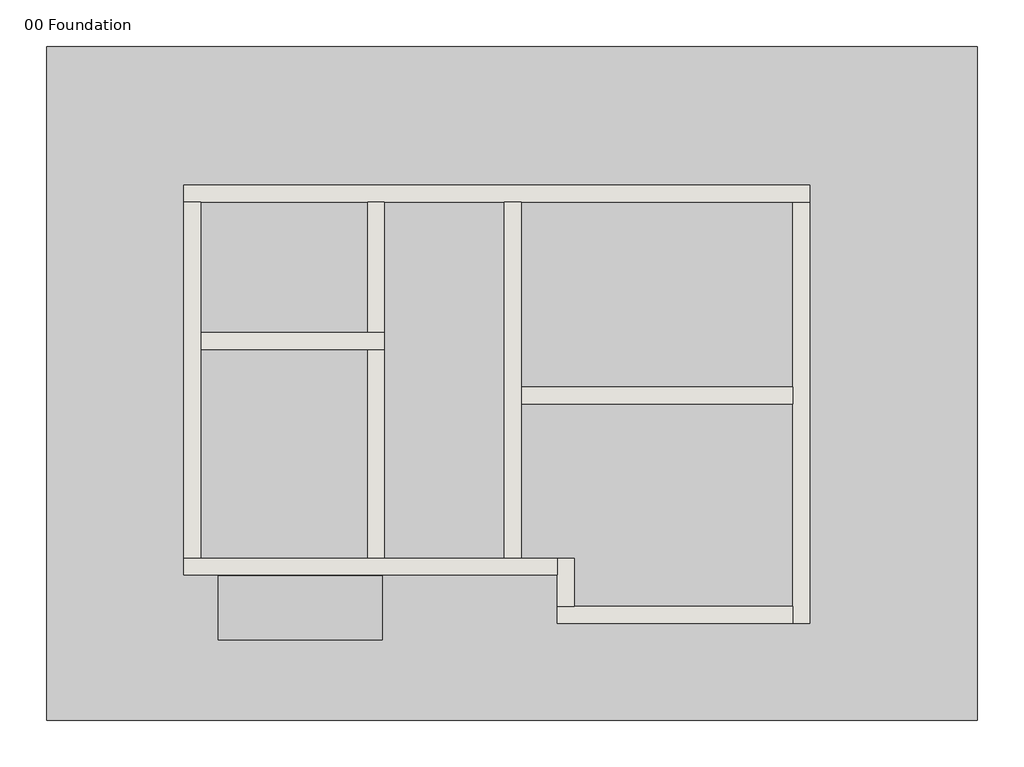
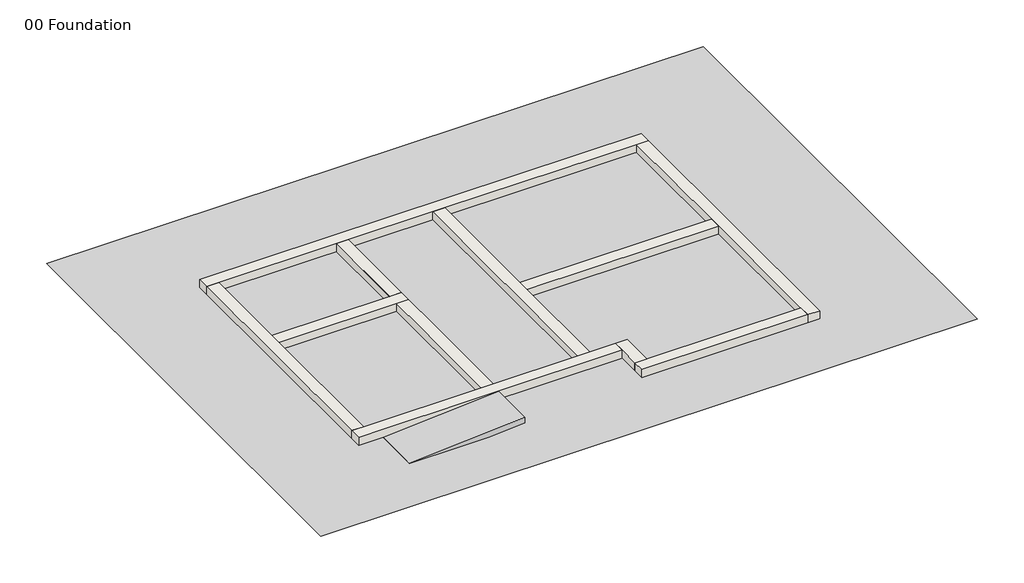
# One storey: 21 walls, 10 footings, 1 proxy, 1 ramp.
"""IFC4 building model written with IfcOpenShell, lengths in millimetres."""

import ifcopenshell
import ifcopenshell.guid

model = None  # the IFC model being written
_history = None  # IfcOwnerHistory: only IFC2X3 demands one
_inside = {}  # id of a spatial element -> (the spatial element, [elements in it])
_under = {}  # id of a project, library or spatial element -> (it, [spatial elements below it])
_declared = {}  # id of a project -> (the project, [libraries it declares])
_typed = {}  # id of a type object -> (the type object, [elements of that type])
_made_of = {}  # id of a material, layer set ... -> (it, [elements and type objects made of it])


def new_model(schema):
    """Start an empty IFC model of exactly this schema.

    Asked for "IFC4X3", IfcOpenShell would pick the latest addendum, in which some entities
    have other attributes; the version numbers below select the first issue.
    IFC2X3 requires an IfcOwnerHistory on every rooted entity: one is made here for all.
    """
    global model, _history
    if schema == "IFC4X3":
        model = ifcopenshell.file(schema_version=(4, 3, 0, 0))
    else:
        model = ifcopenshell.file(schema=schema)
    _inside.clear()
    _under.clear()
    _declared.clear()
    _typed.clear()
    _made_of.clear()
    _history = None
    if model.schema == "IFC2X3":
        org = make("IfcOrganization", Name="unknown")
        user = make(
            "IfcPersonAndOrganization",
            ThePerson=make("IfcPerson", FamilyName="unknown"),
            TheOrganization=org,
        )
        app = make(
            "IfcApplication",
            ApplicationDeveloper=org,
            Version="unknown",
            ApplicationFullName="unknown",
            ApplicationIdentifier="unknown",
        )
        _history = make(
            "IfcOwnerHistory",
            OwningUser=user,
            OwningApplication=app,
            ChangeAction="ADDED",
            CreationDate=0,
        )
    return model


def make(cls, **values):
    """One entity of the class cls with the attributes given. An attribute that is None is left unset."""
    return model.create_entity(
        cls, **{name: value for name, value in values.items() if value is not None}
    )


def rooted(cls, **values):
    """An entity with a GlobalId (a new one), such as an element, a storey or a relation."""
    return make(cls, GlobalId=ifcopenshell.guid.new(), OwnerHistory=_history, **values)


def si_unit(unit_type, name, prefix=None):
    """IfcSIUnit, for example si_unit("LENGTHUNIT", "METRE", prefix="MILLI")."""
    return make("IfcSIUnit", UnitType=unit_type, Prefix=prefix, Name=name)


def assignment(units):
    """IfcUnitAssignment: the units of a project."""
    return None if units is None else make("IfcUnitAssignment", Units=units)


def point(xyz):
    """IfcCartesianPoint."""
    return None if xyz is None else make("IfcCartesianPoint", Coordinates=xyz)


def direction(xyz):
    """IfcDirection."""
    return None if xyz is None else make("IfcDirection", DirectionRatios=xyz)


def frame(location, z_axis=None, x_axis=None):
    """IfcAxis2Placement3D, a coordinate frame: its origin and axes. An axis left out is left unset."""
    return make(
        "IfcAxis2Placement3D",
        Location=point(location),
        Axis=direction(z_axis),
        RefDirection=direction(x_axis),
    )


def origin():
    """The frame at (0, 0, 0) with its axes left unset."""
    return frame((0.0, 0.0, 0.0))


def place(relative_to, where):
    """IfcLocalPlacement: puts the frame where relative to a parent placement (None: the world)."""
    return make(
        "IfcLocalPlacement", PlacementRelTo=relative_to, RelativePlacement=where
    )


def context(
    kind, dimensions, precision=None, world=None, true_north=None, identifier=None
):
    """IfcGeometricRepresentationContext, for example the 3D "Model" context."""
    return make(
        "IfcGeometricRepresentationContext",
        ContextIdentifier=identifier,
        ContextType=kind,
        CoordinateSpaceDimension=dimensions,
        Precision=precision,
        WorldCoordinateSystem=world,
        TrueNorth=true_north,
    )


def project(units=None, contexts=None):
    """IfcProject with its units and contexts."""
    return rooted(
        "IfcProject",
        Name="project",
        RepresentationContexts=contexts,
        UnitsInContext=assignment(units),
    )


def spatial(cls, under=None, at=None, **own):
    """A site, building, storey or space (cls), placed at a placement, below another one or the project."""
    s = rooted(cls, ObjectPlacement=at, **own)
    if under is not None:
        _under.setdefault(under.id(), (under, []))[1].append(s)
    return s


def polyline(points):
    """IfcPolyline through the points."""
    return make("IfcPolyline", Points=[point(p) for p in points])


def point_list(points):
    """IfcCartesianPointList2D or 3D."""
    cls = (
        "IfcCartesianPointList2D" if len(points[0]) == 2 else "IfcCartesianPointList3D"
    )
    return make(cls, CoordList=points)


def outline(outer, holes=None, kind="AREA"):
    """IfcArbitraryClosedProfileDef: a profile drawn as a closed curve; with holes, ...WithVoids."""
    if holes is None:
        return make("IfcArbitraryClosedProfileDef", ProfileType=kind, OuterCurve=outer)
    return make(
        "IfcArbitraryProfileDefWithVoids",
        ProfileType=kind,
        OuterCurve=outer,
        InnerCurves=holes,
    )


def extrude(swept, where, along, depth):
    """IfcExtrudedAreaSolid: the profile swept, set in the frame where, extruded along a direction by depth."""
    return make(
        "IfcExtrudedAreaSolid",
        SweptArea=swept,
        Position=where,
        ExtrudedDirection=direction(along),
        Depth=depth,
    )


def faces_of(points, faces, orient=None, outer=None):
    """IfcFace entities. A face is a list of loops; a loop is a list of indices into points, from 0.

    orient and outer hold one flag for each loop. By default every Orientation is true, the
    first loop of a face is its IfcFaceOuterBound and the others are IfcFaceBound.
    """
    made = []
    for i, loops in enumerate(faces):
        bounds = []
        for j, loop in enumerate(loops):
            is_outer = j == 0 if outer is None else outer[i][j]
            bounds.append(
                make(
                    "IfcFaceOuterBound" if is_outer else "IfcFaceBound",
                    Bound=make("IfcPolyLoop", Polygon=[points[k] for k in loop]),
                    Orientation=True if orient is None else orient[i][j],
                )
            )
        made.append(make("IfcFace", Bounds=bounds))
    return made


def faceted_brep(points, faces, orient=None, outer=None, voids=None):
    """IfcFacetedBrep: a solid bounded by flat faces; with voids (closed shells), ...WithVoids."""
    shared = [point(p) for p in points]
    hull = make("IfcClosedShell", CfsFaces=faces_of(shared, faces, orient, outer))
    if voids is None:
        return make("IfcFacetedBrep", Outer=hull)
    return make(
        "IfcFacetedBrepWithVoids",
        Outer=hull,
        Voids=[
            make(cls, CfsFaces=faces_of(shared, fs, o, b)) for cls, fs, o, b in voids
        ],
    )


def triangles(points, corners, closed=None, point_numbers=None):
    """IfcTriangulatedFaceSet: each triangle names its three corners, points numbered from 1."""
    return make(
        "IfcTriangulatedFaceSet",
        Coordinates=point_list(points),
        Closed=closed,
        CoordIndex=corners,
        PnIndex=point_numbers,
    )


def shape(context_of_items, identifier, shape_type, items):
    """IfcShapeRepresentation: the items that make up one representation, for example the "Body"."""
    return make(
        "IfcShapeRepresentation",
        ContextOfItems=context_of_items,
        RepresentationIdentifier=identifier,
        RepresentationType=shape_type,
        Items=items,
    )


def source(mapping_origin, context_of_items, identifier, shape_type, items):
    """IfcRepresentationMap: a shape defined once, which mapped items show again and again."""
    return make(
        "IfcRepresentationMap",
        MappingOrigin=mapping_origin,
        MappedRepresentation=shape(context_of_items, identifier, shape_type, items),
    )


def transform(
    local_origin,
    x_axis=None,
    y_axis=None,
    z_axis=None,
    scale=None,
    scale2=None,
    scale3=None,
    uniform=True,
):
    """IfcCartesianTransformationOperator3D, or its non-uniform kind. x_axis, y_axis, z_axis: its Axis1, 2, 3."""
    if uniform:
        return make(
            "IfcCartesianTransformationOperator3D",
            Axis1=direction(x_axis),
            Axis2=direction(y_axis),
            LocalOrigin=point(local_origin),
            Scale=scale,
            Axis3=direction(z_axis),
        )
    return make(
        "IfcCartesianTransformationOperator3DnonUniform",
        Axis1=direction(x_axis),
        Axis2=direction(y_axis),
        LocalOrigin=point(local_origin),
        Scale=scale,
        Axis3=direction(z_axis),
        Scale2=scale2,
        Scale3=scale3,
    )


def mapped(mapping_source, mapping_target):
    """IfcMappedItem: shows the shape of a source again, moved by a transform."""
    return make(
        "IfcMappedItem", MappingSource=mapping_source, MappingTarget=mapping_target
    )


def made_of(thing, what):
    """Note that an element or type object is made of a material, layer set ...; save() writes the relation."""
    if what is not None:
        _made_of.setdefault(what.id(), (what, []))[1].append(thing)
    return thing


def element(
    cls,
    number,
    at=None,
    inside=None,
    cuts=None,
    type_object=None,
    material=None,
    context=None,
    identifier="Body",
    shape_type=None,
    held_by="IfcProductDefinitionShape",
    body=None,
    shapes=None,
    **own,
):
    """One element of the class cls, such as IfcWall. Its Tag is "e" and its number.

    at: its placement. inside: the storey or other place that contains it. cuts: it is an
    opening in that element (IfcRelVoidsElement). A single representation is given by context,
    identifier, shape_type and body (its items); several are given by shapes. held_by: the class
    of the entity that holds the representations. save() writes the other relations.
    """
    e = rooted(cls, Tag="e%d" % number, ObjectPlacement=at, **own)
    if body is not None:
        shapes = [shape(context, identifier, shape_type, body)]
    if shapes is not None:
        e.Representation = make(held_by, Representations=shapes)
    if inside is not None:
        _inside.setdefault(inside.id(), (inside, []))[1].append(e)
    if cuts is not None:
        rooted(
            "IfcRelVoidsElement", RelatingBuildingElement=cuts, RelatedOpeningElement=e
        )
    if type_object is not None:
        _typed.setdefault(type_object.id(), (type_object, []))[1].append(e)
    return made_of(e, material)


def aggregate(whole, parts):
    """IfcRelAggregates: a whole, such as a stair, and the parts it consists of."""
    return rooted("IfcRelAggregates", RelatingObject=whole, RelatedObjects=parts)


def save(model, path):
    """Write the relations noted so far, then the file.

    IfcRelAggregates (storeys below a building ...), IfcRelContainedInSpatialStructure (elements
    in a storey), IfcRelDefinesByType, IfcRelAssociatesMaterial and IfcRelDeclares: one each for
    every whole, place, type object, material and project.
    """
    for whole, parts in _under.values():
        aggregate(whole, parts)
    for where, things in _inside.values():
        rooted(
            "IfcRelContainedInSpatialStructure",
            RelatedElements=things,
            RelatingStructure=where,
        )
    for kind, things in _typed.values():
        rooted("IfcRelDefinesByType", RelatedObjects=things, RelatingType=kind)
    for what, things in _made_of.values():
        rooted("IfcRelAssociatesMaterial", RelatedObjects=things, RelatingMaterial=what)
    for by, libraries in _declared.values():
        rooted("IfcRelDeclares", RelatingContext=by, RelatedDefinitions=libraries)
    model.write(path)


def ramp_1_ce501800(model_context):
    return source(origin(), model_context, "Body", "SweptSolid", [
        extrude(outline(polyline([(0.0, -7500.2064028), (-225.0, -10560.2064028), (-375.4049465, -10560.2064028), (-150.4049465, -7500.2064028), (0.0, -7500.2064028)])), frame((0.0, -1636.162817, 0.0), z_axis=(0.0, 1.0, 0.0), x_axis=(0.0, 0.0, 1.0)), (0.0, 0.0, 1.0), 1200.0),
    ])


model = new_model("IFC4")

# Units and contexts
model_context = context("Model", 3, world=origin())
ifc_project = project(units=[si_unit("LENGTHUNIT", "METRE", prefix="MILLI")], contexts=[model_context])

# Site, building, storey
site = spatial("IfcSite", under=ifc_project)
building = spatial("IfcBuilding", under=site)
storey = spatial("IfcBuildingStorey", under=building, Name="00 Foundation", Elevation=-900.0)

# Proxy
placement = place(None, origin())
element("IfcBuildingElementProxy", 1, Name="Building Element Proxy", at=placement, inside=storey, context=model_context, shape_type="Tessellation", body=[
    triangles([(-13772.2558685, 9461.3562103, -225.0000017), (3627.7439735, 9461.3562103, -225.0000017), (3627.7439735, -3138.6435951, -225.0000017), (-13772.2558685, -3138.6435951, -225.0000017)], [[1, 4, 2], [3, 2, 4]], closed=False),
])

# Footings
element("IfcFooting", 2, ObjectType="Wall Foundation Domestic 910", at=placement, inside=storey, context=model_context, shape_type="Brep", body=[
    faceted_brep([(-10595.3997381, -720.6350684, -900.0), (-10595.3997381, 189.3649316, -900.0), (-10595.3997381, 3496.6149316, -900.0), (-10595.3997381, 4406.6149316, -900.0), (-10595.3997381, 6255.1149316, -900.0), (-10595.3997381, 7165.1149316, -900.0), (-11505.3997381, 7165.1149316, -900.0), (-11505.3997381, -720.6350684, -900.0), (-11505.3997381, -720.6350684, -1250.0), (-11505.3997381, 7165.1149316, -1250.0), (-10595.3997381, -720.6350684, -1250.0), (-10595.3997381, 7165.1149316, -1250.0), (-10595.3997381, 6255.1149316, -1250.0), (-10595.3997381, 4406.6149316, -1250.0), (-10595.3997381, 3496.6149316, -1250.0), (-10595.3997381, 189.3649316, -1250.0)], [[[0, 1, 2, 3, 4, 5, 6, 7]], [[8, 7, 6, 9]], [[10, 8, 9, 11, 12, 13, 14, 15]], [[0, 10, 15, 14, 13, 12, 11, 5, 4, 3, 2, 1]], [[6, 5, 11, 9]], [[0, 7, 8, 10]]]),
])
element("IfcFooting", 3, ObjectType="Wall Foundation Domestic 910", at=placement, inside=storey, context=model_context, shape_type="Brep", body=[
    faceted_brep([(792.3502619, 6255.1149316, -900.0), (792.3502619, 7165.1149316, -900.0), (-10595.3997381, 7165.1149316, -900.0), (-10595.3997381, 6255.1149316, -900.0), (-8069.2747381, 6255.1149316, -900.0), (-7159.2747381, 6255.1149316, -900.0), (-5512.2747381, 6255.1149316, -900.0), (-4602.2747381, 6255.1149316, -900.0), (-117.6497381, 6255.1149316, -900.0), (792.3502619, 7165.1149316, -1250.0), (-10595.3997381, 7165.1149316, -1250.0), (792.3502619, 6255.1149316, -1250.0), (-117.6497381, 6255.1149316, -1250.0), (-4602.2747381, 6255.1149316, -1250.0), (-5512.2747381, 6255.1149316, -1250.0), (-7159.2747381, 6255.1149316, -1250.0), (-8069.2747381, 6255.1149316, -1250.0), (-10595.3997381, 6255.1149316, -1250.0)], [[[0, 1, 2, 3, 4, 5, 6, 7, 8]], [[1, 9, 10, 2]], [[9, 11, 12, 13, 14, 15, 16, 17, 10]], [[11, 0, 8, 7, 6, 5, 4, 3, 17, 16, 15, 14, 13, 12]], [[3, 2, 10, 17]], [[1, 0, 11, 9]]]),
])
element("IfcFooting", 4, ObjectType="Wall Foundation Domestic 910", at=placement, inside=storey, context=model_context, shape_type="Brep", body=[
    faceted_brep([(-10595.3997381, 3496.6149316, -900.0), (-8069.2747381, 3496.6149316, -900.0), (-7159.2747381, 3496.6149316, -900.0), (-7159.2747381, 4406.6149316, -900.0), (-8069.2747381, 4406.6149316, -900.0), (-10595.3997381, 4406.6149316, -900.0), (-10595.3997381, 4406.6149316, -1250.0), (-7159.2747381, 4406.6149316, -1250.0), (-8069.2747381, 4406.6149316, -1250.0), (-10595.3997381, 3496.6149316, -1250.0), (-7159.2747381, 3496.6149316, -1250.0), (-8069.2747381, 3496.6149316, -1250.0)], [[[0, 1, 2, 3, 4, 5]], [[6, 5, 4, 3, 7, 8]], [[9, 6, 8, 7, 10, 11]], [[0, 9, 11, 10, 2, 1]], [[0, 5, 6, 9]], [[3, 2, 10, 7]]]),
])
element("IfcFooting", 5, ObjectType="Wall Foundation Domestic 910", at=placement, inside=storey, context=model_context, shape_type="SweptSolid", body=[
    extrude(outline(polyline([(-8069.2747381, 6255.1149316), (-7159.2747381, 6255.1149316), (-7159.2747381, 4406.6149316), (-8069.2747381, 4406.6149316), (-8069.2747381, 6255.1149316)])), frame((0.0, 0.0, -1250.0), z_axis=(0.0, 0.0, 1.0), x_axis=(1.0, 0.0, 0.0)), (0.0, 0.0, 1.0), 350.0),
    extrude(outline(polyline([(-7159.2747381, 189.3649316), (-8069.2747381, 189.3649316), (-8069.2747381, 3496.6149316), (-7159.2747381, 3496.6149316), (-7159.2747381, 189.3649316)])), frame((0.0, 0.0, -1250.0), z_axis=(0.0, 0.0, 1.0), x_axis=(1.0, 0.0, 0.0)), (0.0, 0.0, 1.0), 350.0),
])
element("IfcFooting", 6, ObjectType="Wall Foundation Domestic 910", at=placement, inside=storey, context=model_context, shape_type="Brep", body=[
    faceted_brep([(-5512.2747381, 6255.1149316, -900.0), (-5512.2747381, 189.3649316, -900.0), (-4602.2747381, 189.3649316, -900.0), (-4602.2747381, 2480.3649316, -900.0), (-4602.2747381, 3390.3649316, -900.0), (-4602.2747381, 6255.1149316, -900.0), (-4602.2747381, 6255.1149316, -1250.0), (-4602.2747381, 189.3649316, -1250.0), (-4602.2747381, 2480.3649316, -1250.0), (-4602.2747381, 3390.3649316, -1250.0), (-5512.2747381, 6255.1149316, -1250.0), (-5512.2747381, 189.3649316, -1250.0)], [[[0, 1, 2, 3, 4, 5]], [[6, 5, 4, 3, 2, 7, 8, 9]], [[10, 6, 9, 8, 7, 11]], [[0, 10, 11, 1]], [[0, 5, 6, 10]], [[2, 1, 11, 7]]]),
])
element("IfcFooting", 7, ObjectType="Wall Foundation Domestic 910", at=placement, inside=storey, context=model_context, shape_type="SweptSolid", body=[
    extrude(outline(polyline([(-117.6497381, 3390.3649316), (-117.6497381, 2480.3649316), (-4602.2747381, 2480.3649316), (-4602.2747381, 3390.3649316), (-117.6497381, 3390.3649316)])), frame((0.0, 0.0, -1250.0), z_axis=(0.0, 0.0, 1.0), x_axis=(1.0, 0.0, 0.0)), (0.0, 0.0, 1.0), 350.0),
])
element("IfcFooting", 8, ObjectType="Wall Foundation Domestic 910", at=placement, inside=storey, context=model_context, shape_type="Brep", body=[
    faceted_brep([(-117.6497381, -1620.6350684, -900.0), (792.3502619, -1620.6350684, -900.0), (792.3502619, 6255.1149316, -900.0), (-117.6497381, 6255.1149316, -900.0), (-117.6497381, 3390.3649316, -900.0), (-117.6497381, 2480.3649316, -900.0), (-117.6497381, -710.6350684, -900.0), (792.3502619, -1620.6350684, -1250.0), (792.3502619, 6255.1149316, -1250.0), (-117.6497381, -1620.6350684, -1250.0), (-117.6497381, -710.6350684, -1250.0), (-117.6497381, 2480.3649316, -1250.0), (-117.6497381, 3390.3649316, -1250.0), (-117.6497381, 6255.1149316, -1250.0)], [[[0, 1, 2, 3, 4, 5, 6]], [[1, 7, 8, 2]], [[7, 9, 10, 11, 12, 13, 8]], [[9, 0, 6, 5, 4, 3, 13, 12, 11, 10]], [[3, 2, 8, 13]], [[1, 0, 9, 7]]]),
])
element("IfcFooting", 9, ObjectType="Wall Foundation Domestic 910", at=placement, inside=storey, context=model_context, shape_type="Brep", body=[
    faceted_brep([(-3609.7747381, -720.6350684, -900.0), (-3609.7747381, -710.6350684, -900.0), (-3609.7747381, 189.3649316, -900.0), (-4602.2747381, 189.3649316, -900.0), (-5512.2747381, 189.3649316, -900.0), (-7159.2747381, 189.3649316, -900.0), (-8069.2747381, 189.3649316, -900.0), (-10595.3997381, 189.3649316, -900.0), (-10595.3997381, -720.6350684, -900.0), (-4519.7747381, -720.6350684, -900.0), (-3609.7747381, -720.6350684, -1250.0), (-10595.3997381, -720.6350684, -1250.0), (-4519.7747381, -720.6350684, -1250.0), (-3609.7747381, 189.3649316, -1250.0), (-3609.7747381, -710.6350684, -1250.0), (-10595.3997381, 189.3649316, -1250.0), (-8069.2747381, 189.3649316, -1250.0), (-7159.2747381, 189.3649316, -1250.0), (-5512.2747381, 189.3649316, -1250.0), (-4602.2747381, 189.3649316, -1250.0)], [[[0, 1, 2, 3, 4, 5, 6, 7, 8, 9]], [[10, 0, 9, 8, 11, 12]], [[13, 14, 10, 12, 11, 15, 16, 17, 18, 19]], [[2, 13, 19, 18, 17, 16, 15, 7, 6, 5, 4, 3]], [[8, 7, 15, 11]], [[2, 1, 0, 10, 14, 13]]]),
])
element("IfcFooting", 10, ObjectType="Wall Foundation Domestic 910", at=placement, inside=storey, context=model_context, shape_type="SweptSolid", body=[
    extrude(outline(polyline([(-3609.7747381, -1620.6350684), (-4519.7747381, -1620.6350684), (-4519.7747381, -720.6350684), (-3609.7747381, -720.6350684), (-3609.7747381, -1620.6350684)])), frame((0.0, 0.0, -1250.0), z_axis=(0.0, 0.0, 1.0), x_axis=(1.0, 0.0, 0.0)), (0.0, 0.0, 1.0), 350.0),
])
element("IfcFooting", 11, ObjectType="Wall Foundation Domestic 910", at=placement, inside=storey, context=model_context, shape_type="Brep", body=[
    faceted_brep([(-117.6497381, -1620.6350684, -900.0), (-117.6497381, -710.6350684, -900.0), (-3609.7747381, -710.6350684, -900.0), (-3609.7747381, -720.6350684, -900.0), (-3609.7747381, -1620.6350684, -900.0), (-117.6497381, -1620.6350684, -1250.0), (-3609.7747381, -1620.6350684, -1250.0), (-117.6497381, -710.6350684, -1250.0), (-3609.7747381, -720.6350684, -1250.0), (-3609.7747381, -710.6350684, -1250.0)], [[[0, 1, 2, 3, 4]], [[5, 0, 4, 6]], [[7, 5, 6, 8, 9]], [[1, 7, 9, 2]], [[1, 0, 5, 7]], [[2, 9, 8, 6, 4, 3]]]),
])

# Ramp
ramp_1_shape = ramp_1_ce501800(model_context)
element("IfcRamp", 12, ObjectType="Ramp 1", at=placement, inside=storey, context=model_context, shape_type="MappedRepresentation", body=[
    mapped(ramp_1_shape, transform((0.0, 0.0, 0.0), x_axis=(1.0, 0.0, 0.0), y_axis=(0.0, 1.0, 0.0), z_axis=(0.0, 0.0, 1.0))),
])

# Walls
element("IfcWall", 13, ObjectType="EF_20_05_Wall-Fnd_440DBlk (Trench Blockwork)", at=placement, inside=storey, context=model_context, shape_type="Brep", body=[
    faceted_brep([(-10830.3997381, -45.6350684, -900.0), (-10830.3997381, 3731.6149316, -900.0), (-10830.3997381, 4171.6149316, -900.0), (-10830.3997381, 6490.1149316, -900.0), (-10830.3997381, 6930.1149316, -900.0), (-10830.3997381, 6930.1149316, -450.0), (-10830.3997381, 6490.1149316, -450.0), (-10830.3997381, 4171.6149316, -450.0), (-10830.3997381, 3731.6149316, -450.0), (-10830.3997381, -45.6350684, -450.0), (-11270.3997381, -45.6350684, -900.0), (-11270.3997381, -45.6350684, -450.0), (-11270.3997381, 6930.1149316, -450.0), (-11270.3997381, 6930.1149316, -900.0)], [[[0, 1, 2, 3, 4, 5, 6, 7, 8, 9]], [[10, 11, 12, 13]], [[4, 3, 2, 1, 0, 10, 13]], [[9, 8, 7, 6, 5, 12, 11]], [[5, 4, 13, 12]], [[0, 9, 11, 10]]]),
])
element("IfcWall", 14, ObjectType="EF_20_05_Wall-Fnd_440DBlk (Trench Blockwork)", at=placement, inside=storey, context=model_context, shape_type="Brep", body=[
    faceted_brep([(-10830.3997381, 6490.1149316, -900.0), (-7834.2747381, 6490.1149316, -900.0), (-7394.2747381, 6490.1149316, -900.0), (-5277.2747381, 6490.1149316, -900.0), (-4837.2747381, 6490.1149316, -900.0), (117.3502619, 6490.1149316, -900.0), (557.3502619, 6490.1149316, -900.0), (557.3502619, 6490.1149316, -450.0), (117.3502619, 6490.1149316, -450.0), (-4837.2747381, 6490.1149316, -450.0), (-5277.2747381, 6490.1149316, -450.0), (-7394.2747381, 6490.1149316, -450.0), (-7834.2747381, 6490.1149316, -450.0), (-10830.3997381, 6490.1149316, -450.0), (-10830.3997381, 6930.1149316, -900.0), (-10830.3997381, 6930.1149316, -450.0), (557.3502619, 6930.1149316, -450.0), (557.3502619, 6930.1149316, -900.0)], [[[0, 1, 2, 3, 4, 5, 6, 7, 8, 9, 10, 11, 12, 13]], [[14, 15, 16, 17]], [[6, 5, 4, 3, 2, 1, 0, 14, 17]], [[13, 12, 11, 10, 9, 8, 7, 16, 15]], [[0, 13, 15, 14]], [[7, 6, 17, 16]]]),
])
element("IfcWall", 15, ObjectType="EF_20_05_Wall-Fnd_440DBlk (Trench Blockwork)", at=placement, inside=storey, context=model_context, shape_type="Brep", body=[
    faceted_brep([(117.3502619, 6490.1149316, -900.0), (117.3502619, 3155.3649316, -900.0), (117.3502619, 2715.3649316, -900.0), (117.3502619, -945.6350684, -900.0), (117.3502619, -1385.6350684, -900.0), (117.3502619, -1385.6350684, -450.0), (117.3502619, -945.6350684, -450.0), (117.3502619, 2715.3649316, -450.0), (117.3502619, 3155.3649316, -450.0), (117.3502619, 6490.1149316, -450.0), (557.3502619, 6490.1149316, -900.0), (557.3502619, 6490.1149316, -450.0), (557.3502619, -1385.6350684, -450.0), (557.3502619, -1385.6350684, -900.0)], [[[0, 1, 2, 3, 4, 5, 6, 7, 8, 9]], [[10, 11, 12, 13]], [[4, 3, 2, 1, 0, 10, 13]], [[9, 8, 7, 6, 5, 12, 11]], [[5, 4, 13, 12]], [[0, 9, 11, 10]]]),
])
element("IfcWall", 16, ObjectType="EF_20_05_Wall-Fnd_440DBlk (Trench Blockwork)", at=placement, inside=storey, context=model_context, shape_type="Brep", body=[
    faceted_brep([(-4284.7747381, -45.6350684, -900.0), (-4837.2747381, -45.6350684, -900.0), (-5277.2747381, -45.6350684, -900.0), (-7394.2747381, -45.6350684, -900.0), (-7834.2747381, -45.6350684, -900.0), (-10830.3997381, -45.6350684, -900.0), (-11270.3997381, -45.6350684, -900.0), (-11270.3997381, -45.6350684, -450.0), (-10830.3997381, -45.6350684, -450.0), (-7834.2747381, -45.6350684, -450.0), (-7394.2747381, -45.6350684, -450.0), (-5277.2747381, -45.6350684, -450.0), (-4837.2747381, -45.6350684, -450.0), (-4284.7747381, -45.6350684, -450.0), (-4284.7747381, -485.6350684, -900.0), (-4284.7747381, -485.6350684, -450.0), (-11270.3997381, -485.6350684, -450.0), (-11270.3997381, -485.6350684, -900.0)], [[[0, 1, 2, 3, 4, 5, 6, 7, 8, 9, 10, 11, 12, 13]], [[14, 15, 16, 17]], [[6, 5, 4, 3, 2, 1, 0, 14, 17]], [[13, 12, 11, 10, 9, 8, 7, 16, 15]], [[7, 6, 17, 16]], [[0, 13, 15, 14]]]),
])
element("IfcWall", 17, ObjectType="EF_20_05_Wall-Fnd_440DBlk (Trench Blockwork)", at=placement, inside=storey, context=model_context, shape_type="SweptSolid", body=[
    extrude(outline(polyline([(-3844.7747381, -945.6350684), (117.3502619, -945.6350684), (117.3502619, -1385.6350684), (-3844.7747381, -1385.6350684), (-3844.7747381, -945.6350684)])), frame((0.0, 0.0, -900.0), z_axis=(0.0, 0.0, 1.0), x_axis=(1.0, 0.0, 0.0)), (0.0, 0.0, 1.0), 450.0),
])
element("IfcWall", 18, ObjectType="EF_20_05_Wall-Fnd_440DBlk (Trench Blockwork)", at=placement, inside=storey, context=model_context, shape_type="Brep", body=[
    faceted_brep([(-3844.7747381, -1385.6350684, -900.0), (-3844.7747381, -945.6350684, -900.0), (-3844.7747381, -45.6350684, -900.0), (-3844.7747381, -45.6350684, -450.0), (-3844.7747381, -945.6350684, -450.0), (-3844.7747381, -1385.6350684, -450.0), (-4284.7747381, -1385.6350684, -900.0), (-4284.7747381, -1385.6350684, -450.0), (-4284.7747381, -485.6350684, -450.0), (-4284.7747381, -45.6350684, -450.0), (-4284.7747381, -45.6350684, -900.0), (-4284.7747381, -485.6350684, -900.0)], [[[0, 1, 2, 3, 4, 5]], [[6, 7, 8, 9, 10, 11]], [[2, 1, 0, 6, 11, 10]], [[5, 4, 3, 9, 8, 7]], [[3, 2, 10, 9]], [[0, 5, 7, 6]]]),
])
element("IfcWall", 19, ObjectType="EF_20_05_Wall-Fnd_440DBlk (Trench Blockwork)", at=placement, inside=storey, context=model_context, shape_type="SweptSolid", body=[
    extrude(outline(polyline([(-7834.2747381, 3731.6149316), (-10830.3997381, 3731.6149316), (-10830.3997381, 4171.6149316), (-7834.2747381, 4171.6149316), (-7834.2747381, 3731.6149316)])), frame((0.0, 0.0, -900.0), z_axis=(0.0, 0.0, 1.0), x_axis=(1.0, 0.0, 0.0)), (0.0, 0.0, 1.0), 450.0),
])
element("IfcWall", 20, ObjectType="EF_20_05_Wall-Fnd_440DBlk (Trench Blockwork)", at=placement, inside=storey, context=model_context, shape_type="Brep", body=[
    faceted_brep([(-7394.2747381, -45.6350684, -900.0), (-7394.2747381, 6490.1149316, -900.0), (-7394.2747381, 6490.1149316, -450.0), (-7394.2747381, -45.6350684, -450.0), (-7834.2747381, -45.6350684, -900.0), (-7834.2747381, -45.6350684, -450.0), (-7834.2747381, 3731.6149316, -450.0), (-7834.2747381, 4171.6149316, -450.0), (-7834.2747381, 6490.1149316, -450.0), (-7834.2747381, 6490.1149316, -900.0), (-7834.2747381, 4171.6149316, -900.0), (-7834.2747381, 3731.6149316, -900.0)], [[[0, 1, 2, 3]], [[4, 5, 6, 7, 8, 9, 10, 11]], [[1, 0, 4, 11, 10, 9]], [[3, 2, 8, 7, 6, 5]], [[2, 1, 9, 8]], [[0, 3, 5, 4]]]),
])
element("IfcWall", 21, ObjectType="EF_20_05_Wall-Fnd_440DBlk (Trench Blockwork)", at=placement, inside=storey, context=model_context, shape_type="Brep", body=[
    faceted_brep([(-5277.2747381, 6490.1149316, -900.0), (-5277.2747381, -45.6350684, -900.0), (-5277.2747381, -45.6350684, -450.0), (-5277.2747381, 6490.1149316, -450.0), (-4837.2747381, 6490.1149316, -900.0), (-4837.2747381, 6490.1149316, -450.0), (-4837.2747381, 3155.3649316, -450.0), (-4837.2747381, 2715.3649316, -450.0), (-4837.2747381, -45.6350684, -450.0), (-4837.2747381, -45.6350684, -900.0), (-4837.2747381, 2715.3649316, -900.0), (-4837.2747381, 3155.3649316, -900.0)], [[[0, 1, 2, 3]], [[4, 5, 6, 7, 8, 9, 10, 11]], [[1, 0, 4, 11, 10, 9]], [[3, 2, 8, 7, 6, 5]], [[0, 3, 5, 4]], [[2, 1, 9, 8]]]),
])
element("IfcWall", 22, ObjectType="EF_20_05_Wall-Fnd_440DBlk (Trench Blockwork)", at=placement, inside=storey, context=model_context, shape_type="SweptSolid", body=[
    extrude(outline(polyline([(117.3502619, 2715.3649316), (-4837.2747381, 2715.3649316), (-4837.2747381, 3155.3649316), (117.3502619, 3155.3649316), (117.3502619, 2715.3649316)])), frame((0.0, 0.0, -900.0), z_axis=(0.0, 0.0, 1.0), x_axis=(1.0, 0.0, 0.0)), (0.0, 0.0, 1.0), 450.0),
])
element("IfcWall", 23, ObjectType="EF_25_10_25_Wall-Ext-Cav_100Blk-115Conc-100Blk", at=placement, inside=storey, context=model_context, shape_type="Brep", body=[
    faceted_brep([(-11207.8997381, 6552.6149316, -450.0), (-10892.8997381, 6552.6149316, -450.0), (-7771.7747381, 6552.6149316, -450.0), (-7456.7747381, 6552.6149316, -450.0), (-5214.7747381, 6552.6149316, -450.0), (-4899.7747381, 6552.6149316, -450.0), (179.8502619, 6552.6149316, -450.0), (494.8502619, 6552.6149316, -450.0), (494.8502619, 6552.6149316, 0.0), (179.8502619, 6552.6149316, 0.0), (-4899.7747381, 6552.6149316, 0.0), (-5214.7747381, 6552.6149316, 0.0), (-7456.7747381, 6552.6149316, 0.0), (-7771.7747381, 6552.6149316, 0.0), (-10892.8997381, 6552.6149316, 0.0), (-11207.8997381, 6552.6149316, 0.0), (-11207.8997381, 6867.6149316, -450.0), (-11207.8997381, 6867.6149316, 0.0), (494.8502619, 6867.6149316, 0.0), (494.8502619, 6867.6149316, -450.0)], [[[0, 1, 2, 3, 4, 5, 6, 7, 8, 9, 10, 11, 12, 13, 14, 15]], [[16, 17, 18, 19]], [[7, 6, 5, 4, 3, 2, 1, 0, 16, 19]], [[15, 14, 13, 12, 11, 10, 9, 8, 18, 17]], [[8, 7, 19, 18]], [[0, 15, 17, 16]]]),
])
element("IfcWall", 24, ObjectType="EF_25_10_25_Wall-Ext-Cav_100Blk-115Conc-100Blk", at=placement, inside=storey, context=model_context, shape_type="Brep", body=[
    faceted_brep([(179.8502619, 6552.6149316, -450.0), (179.8502619, 3092.8649316, -450.0), (179.8502619, 2777.8649316, -450.0), (179.8502619, -1008.1350684, -450.0), (179.8502619, -1323.1350684, -450.0), (179.8502619, -1323.1350684, 0.0), (179.8502619, -1008.1350684, 0.0), (179.8502619, 2777.8649316, 0.0), (179.8502619, 3092.8649316, 0.0), (179.8502619, 6552.6149316, 0.0), (494.8502619, 6552.6149316, -450.0), (494.8502619, 6552.6149316, 0.0), (494.8502619, -1323.1350684, 0.0), (494.8502619, -1323.1350684, -450.0)], [[[0, 1, 2, 3, 4, 5, 6, 7, 8, 9]], [[10, 11, 12, 13]], [[4, 3, 2, 1, 0, 10, 13]], [[9, 8, 7, 6, 5, 12, 11]], [[0, 9, 11, 10]], [[5, 4, 13, 12]]]),
])
element("IfcWall", 25, ObjectType="EF_25_10_25_Wall-Ext-Cav_100Blk-115Conc-100Blk", at=placement, inside=storey, context=model_context, shape_type="Brep", body=[
    faceted_brep([(179.8502619, -1008.1350684, -450.0), (-3907.2747381, -1008.1350684, -450.0), (-4222.2747381, -1008.1350684, -450.0), (-4222.2747381, -1008.1350684, 0.0), (-3907.2747381, -1008.1350684, 0.0), (179.8502619, -1008.1350684, 0.0), (179.8502619, -1323.1350684, -450.0), (179.8502619, -1323.1350684, 0.0), (-4222.2747381, -1323.1350684, 0.0), (-4222.2747381, -1323.1350684, -450.0)], [[[0, 1, 2, 3, 4, 5]], [[6, 7, 8, 9]], [[2, 1, 0, 6, 9]], [[5, 4, 3, 8, 7]], [[0, 5, 7, 6]], [[3, 2, 9, 8]]]),
])
element("IfcWall", 26, ObjectType="EF_25_10_25_Wall-Ext-Cav_100Blk-115Conc-100Blk", at=placement, inside=storey, context=model_context, shape_type="Brep", body=[
    faceted_brep([(-3907.2747381, -1008.1350684, -450.0), (-3907.2747381, -108.1350684, -450.0), (-3907.2747381, -108.1350684, 0.0), (-3907.2747381, -1008.1350684, 0.0), (-4222.2747381, -1008.1350684, -450.0), (-4222.2747381, -1008.1350684, 0.0), (-4222.2747381, -423.1350684, 0.0), (-4222.2747381, -108.1350684, 0.0), (-4222.2747381, -108.1350684, -450.0), (-4222.2747381, -423.1350684, -450.0)], [[[0, 1, 2, 3]], [[4, 5, 6, 7, 8, 9]], [[1, 0, 4, 9, 8]], [[3, 2, 7, 6, 5]], [[0, 3, 5, 4]], [[2, 1, 8, 7]]]),
])
element("IfcWall", 27, ObjectType="EF_25_10_25_Wall-Ext-Cav_100Blk-115Conc-100Blk", at=placement, inside=storey, context=model_context, shape_type="Brep", body=[
    faceted_brep([(-4222.2747381, -108.1350684, -450.0), (-4899.7747381, -108.1350684, -450.0), (-5214.7747381, -108.1350684, -450.0), (-7456.7747381, -108.1350684, -450.0), (-7771.7747381, -108.1350684, -450.0), (-10892.8997381, -108.1350684, -450.0), (-11207.8997381, -108.1350684, -450.0), (-11207.8997381, -108.1350684, 0.0), (-10892.8997381, -108.1350684, 0.0), (-7771.7747381, -108.1350684, 0.0), (-7456.7747381, -108.1350684, 0.0), (-5214.7747381, -108.1350684, 0.0), (-4899.7747381, -108.1350684, 0.0), (-4222.2747381, -108.1350684, 0.0), (-4222.2747381, -423.1350684, -450.0), (-4222.2747381, -423.1350684, 0.0), (-11207.8997381, -423.1350684, 0.0), (-11207.8997381, -423.1350684, -450.0)], [[[0, 1, 2, 3, 4, 5, 6, 7, 8, 9, 10, 11, 12, 13]], [[14, 15, 16, 17]], [[6, 5, 4, 3, 2, 1, 0, 14, 17]], [[13, 12, 11, 10, 9, 8, 7, 16, 15]], [[0, 13, 15, 14]], [[7, 6, 17, 16]]]),
])
element("IfcWall", 28, ObjectType="EF_25_10_25_Wall-Ext-Cav_100Blk-115Conc-100Blk", at=placement, inside=storey, context=model_context, shape_type="Brep", body=[
    faceted_brep([(-10892.8997381, -108.1350684, -450.0), (-10892.8997381, 3794.1149316, -450.0), (-10892.8997381, 4109.1149316, -450.0), (-10892.8997381, 6552.6149316, -450.0), (-10892.8997381, 6552.6149316, 0.0), (-10892.8997381, 4109.1149316, 0.0), (-10892.8997381, 3794.1149316, 0.0), (-10892.8997381, -108.1350684, 0.0), (-11207.8997381, -108.1350684, -450.0), (-11207.8997381, -108.1350684, 0.0), (-11207.8997381, 6552.6149316, 0.0), (-11207.8997381, 6552.6149316, -450.0)], [[[0, 1, 2, 3, 4, 5, 6, 7]], [[8, 9, 10, 11]], [[3, 2, 1, 0, 8, 11]], [[7, 6, 5, 4, 10, 9]], [[0, 7, 9, 8]], [[4, 3, 11, 10]]]),
])
element("IfcWall", 29, ObjectType="EF_25_10_25_Wall-Ext-Cav_100Blk-115Conc-100Blk", at=placement, inside=storey, context=model_context, shape_type="Brep", body=[
    faceted_brep([(-10892.8997381, 3794.1149316, -450.0), (-7456.7747381, 3794.1149316, -450.0), (-7456.7747381, 3794.1149316, 0.0), (-10892.8997381, 3794.1149316, 0.0), (-10892.8997381, 4109.1149316, -450.0), (-10892.8997381, 4109.1149316, 0.0), (-7771.7747381, 4109.1149316, 0.0), (-7456.7747381, 4109.1149316, 0.0), (-7456.7747381, 4109.1149316, -450.0), (-7771.7747381, 4109.1149316, -450.0)], [[[0, 1, 2, 3]], [[4, 5, 6, 7, 8, 9]], [[1, 0, 4, 9, 8]], [[3, 2, 7, 6, 5]], [[0, 3, 5, 4]], [[2, 1, 8, 7]]]),
])
element("IfcWall", 30, ObjectType="EF_25_10_25_Wall-Ext-Cav_100Blk-115Conc-100Blk", at=placement, inside=storey, context=model_context, shape_type="SweptSolid", body=[
    extrude(outline(polyline([(-7456.7747381, 6552.6149316), (-7456.7747381, 4109.1149316), (-7771.7747381, 4109.1149316), (-7771.7747381, 6552.6149316), (-7456.7747381, 6552.6149316)])), frame((0.0, 0.0, -450.0), z_axis=(0.0, 0.0, 1.0), x_axis=(1.0, 0.0, 0.0)), (0.0, 0.0, 1.0), 450.0),
])
element("IfcWall", 31, ObjectType="EF_25_10_25_Wall-Ext-Cav_100Blk-115Conc-100Blk", at=placement, inside=storey, context=model_context, shape_type="SweptSolid", body=[
    extrude(outline(polyline([(-7771.7747381, -108.1350684), (-7771.7747381, 6552.6149316), (-7456.7747381, 6552.6149316), (-7456.7747381, -108.1350684), (-7771.7747381, -108.1350684)])), frame((0.0, 0.0, -450.0), z_axis=(0.0, 0.0, 1.0), x_axis=(1.0, 0.0, 0.0)), (0.0, 0.0, 1.0), 450.0),
])
element("IfcWall", 32, ObjectType="EF_25_10_25_Wall-Ext-Cav_100Blk-115Conc-100Blk", at=placement, inside=storey, context=model_context, shape_type="Brep", body=[
    faceted_brep([(-5214.7747381, 6552.6149316, -450.0), (-5214.7747381, -108.1350684, -450.0), (-5214.7747381, -108.1350684, 0.0), (-5214.7747381, 6552.6149316, 0.0), (-4899.7747381, 6552.6149316, -450.0), (-4899.7747381, 6552.6149316, 0.0), (-4899.7747381, 3092.8649316, 0.0), (-4899.7747381, 2777.8649316, 0.0), (-4899.7747381, -108.1350684, 0.0), (-4899.7747381, -108.1350684, -450.0), (-4899.7747381, 2777.8649316, -450.0), (-4899.7747381, 3092.8649316, -450.0)], [[[0, 1, 2, 3]], [[4, 5, 6, 7, 8, 9, 10, 11]], [[1, 0, 4, 11, 10, 9]], [[3, 2, 8, 7, 6, 5]], [[0, 3, 5, 4]], [[2, 1, 9, 8]]]),
])
element("IfcWall", 33, ObjectType="EF_25_10_25_Wall-Ext-Cav_100Blk-115Conc-100Blk", at=placement, inside=storey, context=model_context, shape_type="SweptSolid", body=[
    extrude(outline(polyline([(179.8502619, 2777.8649316), (-4899.7747381, 2777.8649316), (-4899.7747381, 3092.8649316), (179.8502619, 3092.8649316), (179.8502619, 2777.8649316)])), frame((0.0, 0.0, -450.0), z_axis=(0.0, 0.0, 1.0), x_axis=(1.0, 0.0, 0.0)), (0.0, 0.0, 1.0), 450.0),
])

save(model, "model.ifc")

# Revit data of these elements
# Project information
#   Document_Suitability_Code = "P2"
#   Document_Suitability_Description = "Coordination"
#   Project Issue Date = "22-Feb-23"
#   Project Status = "Project Status"
#   Client Name = "Revit Project"
#   Project Address = "Enter address here"
#   Project Name = "Two Storey House"
#   Project Number = "CADD06021-01"
# Type "Ramp 1"
#   built-in parameter 1008304 = 0.492126 (stored number, unit not read)
#   built-in parameter 1008303 = 39.3701 (stored number, unit not read)
#   built-in parameter 1008301 = 12 (stored number, unit not read)
#   Function = 1
#   built-in parameter 1008308 = Concrete, Cast In Situ
# Type "EF_20_05_Wall-Fnd_440DBlk (Trench Blockwork)"
#   Keynote = "F10"
#   Layers, outside or top first: 440 mm "Concrete Masonry Units 440" (function 1)
# Type "EF_25_10_25_Wall-Ext-Cav_100Blk-115Conc-100Blk"
#   Keynote = "F10"
#   Layers, outside or top first: 100 mm "Concrete Masonry Units" (function 4); 115 mm "Concrete, Cast In Situ" (function 3); 100 mm "Concrete Masonry Units" (function 1)
# Element 1 (IfcBuildingElementProxy)
#   Material = Earth
#   Phase Created = New Construction
# Elements 2, 3, 4, 5, 6, 7, 8, 9, 10, 11 (IfcFooting, "Wall Foundation Domestic 910")
#   Comments = ""
#   Phase Created = New Construction
#   Materials on its faces: "Concrete, Cast In Situ"
# Element 12 (IfcRamp, "Ramp 1")
#   built-in parameter 1007275 = "DN"
#   built-in parameter 1007272 = "UP"
#   built-in parameter 1007218 = -0.738189 (stored number, unit not read)
#   Width = 1200 mm
#   built-in parameter 1007276 = 1
#   built-in parameter 1007274 = 1
#   built-in parameter 1007273 = 1
#   built-in parameter 1007271 = 1
#   Phase Created = New Construction
#   Materials on its faces: "Concrete, Cast In Situ"
# Elements 13, 14, 15, 16, 17, 18, 19, 20, 21, 22 (IfcWall, "EF_20_05_Wall-Fnd_440DBlk (Trench Blockwork)")
#   Top Offset = -450 mm
#   Base Offset = 0 mm
#   wall height = 450 mm
#   Phase Created = New Construction
#   Base Constraint = 00 Foundation
#   Top Constraint = 00 Ground Floor
#   Materials on its faces: "Concrete Masonry Units 440"
# Elements 23, 24, 25, 26, 27, 29 (IfcWall, "EF_25_10_25_Wall-Ext-Cav_100Blk-115Conc-100Blk")
#   built-in parameter 1001111 = 450 mm
#   Top Offset = 0 mm
#   Base Offset = 450 mm
#   wall height = 450 mm
#   Phase Created = New Construction
#   Base Constraint = 00 Foundation
#   Top Constraint = 00 Ground Floor
#   Materials on its faces: "Concrete Masonry Units", "Default Wall"
# Elements 28, 30, 31, 32, 33 (IfcWall, "EF_25_10_25_Wall-Ext-Cav_100Blk-115Conc-100Blk")
#   built-in parameter 1001111 = 450 mm
#   Top Offset = 0 mm
#   Base Offset = 450 mm
#   wall height = 450 mm
#   Phase Created = New Construction
#   Base Constraint = 00 Foundation
#   Top Constraint = 00 Ground Floor
#   Materials on its faces: "Default Wall", "Concrete Masonry Units"
# Materials
#   "Concrete, Cast In Situ": class "Concrete", colour RGB 192 192 192, transparency 0, Keynote = "F30/110", Description = "physical material", Cost = 0
#   "Concrete Masonry Units 440": class "Masonry", colour RGB 152 154 138, transparency 0, Keynote = "F10/350", Description = "Concrete masonry units", Cost = 0
#   "Concrete Masonry Units": class "Masonry", colour RGB 117 117 109, transparency 0, Keynote = "F10/350", Description = "Concrete masonry units", Cost = 0
#   "Earth": class "Generic", colour RGB 97 75 62, transparency 0, Description = "Soil", Cost = 0
#   "Default Wall": class "Miscellaneous", colour RGB 128 128 128, transparency 0, Comments = "Rendering appearance not upgraded "
